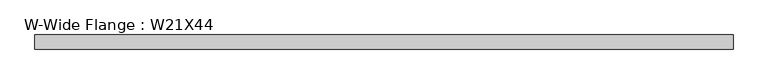
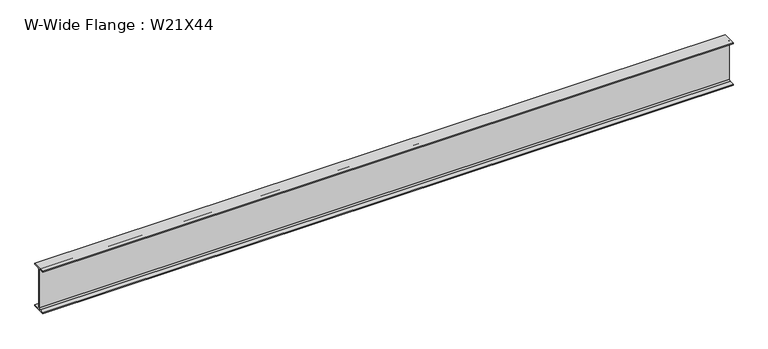
"""IFC4 building model written with IfcOpenShell, lengths in millimetres: beam geometry, W-Wide Flange : W21X44."""

from ifc_helpers import new_model, si_unit, point, frame, frame_2d, origin, place, context, project, spatial, polyline, circle_curve, trimmed, segment, composite_curve, outline, extrude, source, transform, mapped, element, save


def w_wide_flange_w21x44_ac43757c(model_context):
    return source(origin(), model_context, "Body", "SweptSolid", [
        extrude(outline(composite_curve([segment(polyline([(82.55, -251.46), (82.55, -262.89), (-82.55, -262.89), (-82.55, -251.46), (-21.59, -251.46)]), True, "CONTINUOUS"), segment(trimmed(circle_curve(frame_2d((-21.59, -234.315)), 17.145), [point((-21.59, -251.46))], [point((-4.445, -234.315))], True, "CARTESIAN"), True, "CONTINUOUS"), segment(polyline([(-4.445, -234.315), (-4.445, 234.315)]), True, "CONTINUOUS"), segment(trimmed(circle_curve(frame_2d((-21.59, 234.315)), 17.145), [point((-4.445, 234.315))], [point((-21.59, 251.46))], True, "CARTESIAN"), True, "CONTINUOUS"), segment(polyline([(-21.59, 251.46), (-82.55, 251.46), (-82.55, 262.89), (82.55, 262.89), (82.55, 251.46), (21.59, 251.46)]), True, "CONTINUOUS"), segment(trimmed(circle_curve(frame_2d((21.59, 234.315)), 17.145), [point((21.59, 251.46))], [point((4.445, 234.315))], True, "CARTESIAN"), True, "CONTINUOUS"), segment(polyline([(4.445, 234.315), (4.445, -234.315)]), True, "CONTINUOUS"), segment(trimmed(circle_curve(frame_2d((21.59, -234.315)), 17.145), [point((4.445, -234.315))], [point((21.59, -251.46))], True, "CARTESIAN"), True, "CONTINUOUS"), segment(polyline([(21.59, -251.46), (82.55, -251.46)]), True, "CONTINUOUS")], self_intersect=False)), frame((-4105.2253906, 0.0, 0.0), z_axis=(1.0, 0.0, 0.0), x_axis=(0.0, 1.0, 0.0)), (0.0, 0.0, 1.0), 8138.2195313),
    ])


if __name__ == "__main__":
    model = new_model("IFC4")
    model_context = context("Model", 3, world=origin())
    ifc_project = project(units=[si_unit("LENGTHUNIT", "METRE", prefix="MILLI")], contexts=[model_context])
    site = spatial("IfcSite", under=ifc_project)
    building = spatial("IfcBuilding", under=site)
    placement = place(None, origin())
    w_wide_flange_w21x44_shape = w_wide_flange_w21x44_ac43757c(model_context)
    element("IfcBeam", 1, ObjectType="W-Wide Flange : W21X44", at=placement, inside=building, context=model_context, shape_type="MappedRepresentation", body=[
        mapped(w_wide_flange_w21x44_shape, transform((0.0, 0.0, 0.0), x_axis=(1.0, 0.0, 0.0), y_axis=(0.0, 1.0, 0.0), z_axis=(0.0, 0.0, 1.0))),
    ])
    save(model, "model.ifc")

# Revit data of these elements
# Type "W-Wide Flange : W21X44"
#   Assembly Code = "B10"
#   W = 44
#   Length [instance default] = 1524 mm
#   bf = 165.1 mm
#   d = 525.78 mm
#   k = 28.575 mm
#   k2 = 17.145 mm
#   tf = 11.43 mm
#   tw = 8.89 mm
#   A = 0.00838708 m²
#   Structural Material [instance default] = Steel ASTM A992
# Element 1 (IfcBeam, "W-Wide Flange : W21X44")
#   Structural Material = Aluminum, Anodized Red
#   Materials on its faces: "Aluminum, Anodized Red"
# Materials
#   "Steel ASTM A992": class "Metal", colour RGB 128 0 0, transparency 0, Description = "Structural steel 50ksi", Cost = 0
#   "Aluminum, Anodized Red": class "Metal", colour RGB 120 120 120, transparency 0, Description = "Anodized aluminum, red", Cost = 0
